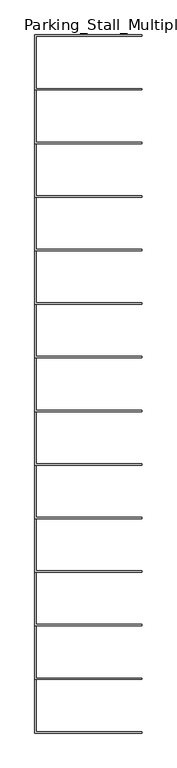
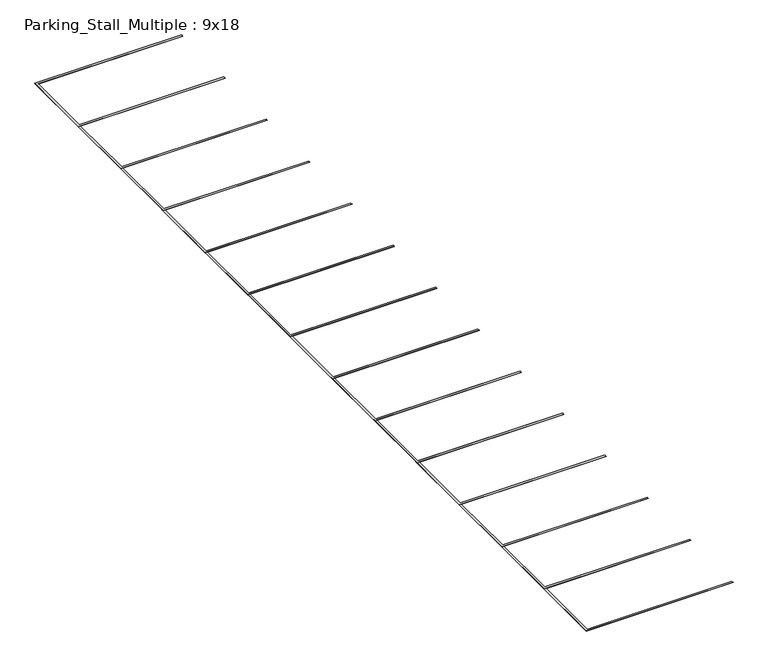
"""IFC4 building model written with IfcOpenShell, lengths in millimetres: proxy geometry, Parking_Stall_Multiple : 9x18."""

from ifc_helpers import new_model, si_unit, origin, origin_with_axes, place, context, project, spatial, polyline, outline, extrude, source, transform, mapped, element, save


def parking_stall_multiple_9x18_8b25bb00(model_context):
    return source(origin(), model_context, "Body", "SweptSolid", [
        extrude(outline(polyline([(5486.4, 32918.4), (0.0, 32918.4), (0.0, 35737.8), (5486.4, 35737.8), (5486.4, 35661.6), (76.2, 35661.6), (76.2, 32994.6), (5486.4, 32994.6), (5486.4, 32918.4)])), origin_with_axes(), (0.0, 0.0, 1.0), 6.35),
        extrude(outline(polyline([(5486.4, 30175.2), (0.0, 30175.2), (0.0, 32994.6), (5486.4, 32994.6), (5486.4, 32918.4), (76.2, 32918.4), (76.2, 30251.4), (5486.4, 30251.4), (5486.4, 30175.2)])), origin_with_axes(), (0.0, 0.0, 1.0), 6.35),
        extrude(outline(polyline([(5486.4, 27432.0), (0.0, 27432.0), (0.0, 30251.4), (5486.4, 30251.4), (5486.4, 30175.2), (76.2, 30175.2), (76.2, 27508.2), (5486.4, 27508.2), (5486.4, 27432.0)])), origin_with_axes(), (0.0, 0.0, 1.0), 6.35),
        extrude(outline(polyline([(5486.4, 24688.8), (0.0, 24688.8), (0.0, 27508.2), (5486.4, 27508.2), (5486.4, 27432.0), (76.2, 27432.0), (76.2, 24765.0), (5486.4, 24765.0), (5486.4, 24688.8)])), origin_with_axes(), (0.0, 0.0, 1.0), 6.35),
        extrude(outline(polyline([(5486.4, 21945.6), (0.0, 21945.6), (0.0, 24765.0), (5486.4, 24765.0), (5486.4, 24688.8), (76.2, 24688.8), (76.2, 22021.8), (5486.4, 22021.8), (5486.4, 21945.6)])), origin_with_axes(), (0.0, 0.0, 1.0), 6.35),
        extrude(outline(polyline([(5486.4, 19202.4), (0.0, 19202.4), (0.0, 22021.8), (5486.4, 22021.8), (5486.4, 21945.6), (76.2, 21945.6), (76.2, 19278.6), (5486.4, 19278.6), (5486.4, 19202.4)])), origin_with_axes(), (0.0, 0.0, 1.0), 6.35),
        extrude(outline(polyline([(5486.4, 16459.2), (0.0, 16459.2), (0.0, 19278.6), (5486.4, 19278.6), (5486.4, 19202.4), (76.2, 19202.4), (76.2, 16535.4), (5486.4, 16535.4), (5486.4, 16459.2)])), origin_with_axes(), (0.0, 0.0, 1.0), 6.35),
        extrude(outline(polyline([(5486.4, 13716.0), (0.0, 13716.0), (0.0, 16535.4), (5486.4, 16535.4), (5486.4, 16459.2), (76.2, 16459.2), (76.2, 13792.2), (5486.4, 13792.2), (5486.4, 13716.0)])), origin_with_axes(), (0.0, 0.0, 1.0), 6.35),
        extrude(outline(polyline([(5486.4, 10972.8), (0.0, 10972.8), (0.0, 13792.2), (5486.4, 13792.2), (5486.4, 13716.0), (76.2, 13716.0), (76.2, 11049.0), (5486.4, 11049.0), (5486.4, 10972.8)])), origin_with_axes(), (0.0, 0.0, 1.0), 6.35),
        extrude(outline(polyline([(5486.4, 8229.6), (0.0, 8229.6), (0.0, 11049.0), (5486.4, 11049.0), (5486.4, 10972.8), (76.2, 10972.8), (76.2, 8305.8), (5486.4, 8305.8), (5486.4, 8229.6)])), origin_with_axes(), (0.0, 0.0, 1.0), 6.35),
        extrude(outline(polyline([(5486.4, 5486.4), (0.0, 5486.4), (0.0, 8305.8), (5486.4, 8305.8), (5486.4, 8229.6), (76.2, 8229.6), (76.2, 5562.6), (5486.4, 5562.6), (5486.4, 5486.4)])), origin_with_axes(), (0.0, 0.0, 1.0), 6.35),
        extrude(outline(polyline([(5486.4, 2743.2), (0.0, 2743.2), (0.0, 5562.6), (5486.4, 5562.6), (5486.4, 5486.4), (76.2, 5486.4), (76.2, 2819.4), (5486.4, 2819.4), (5486.4, 2743.2)])), origin_with_axes(), (0.0, 0.0, 1.0), 6.35),
        extrude(outline(polyline([(5486.4, 0.0), (0.0, 0.0), (0.0, 2819.4), (5486.4, 2819.4), (5486.4, 2743.2), (76.2, 2743.2), (76.2, 76.2), (5486.4, 76.2), (5486.4, 0.0)])), origin_with_axes(), (0.0, 0.0, 1.0), 6.35),
    ])


if __name__ == "__main__":
    model = new_model("IFC4")
    model_context = context("Model", 3, world=origin())
    ifc_project = project(units=[si_unit("LENGTHUNIT", "METRE", prefix="MILLI")], contexts=[model_context])
    site = spatial("IfcSite", under=ifc_project)
    building = spatial("IfcBuilding", under=site)
    placement = place(None, origin())
    parking_stall_multiple_9x18_shape = parking_stall_multiple_9x18_8b25bb00(model_context)
    element("IfcBuildingElementProxy", 1, Name="Parking_Stall_Multiple : 9x18", ObjectType="Parking_Stall_Multiple : 9x18", at=placement, inside=building, context=model_context, shape_type="MappedRepresentation", body=[
        mapped(parking_stall_multiple_9x18_shape, transform((0.0, 0.0, 0.0), x_axis=(1.0, 0.0, 0.0), y_axis=(0.0, 1.0, 0.0), z_axis=(0.0, 0.0, 1.0))),
    ])
    save(model, "model.ifc")

# Revit data of these elements
# Type "Parking_Stall_Multiple : 9x18"
#   Parking_Width_M = 9' - 0"
#   Parking_Run_Length [instance default] = 65' - 0"
#   Parking_Line_Width = 0' - 3"
#   Parking_Length_M = 18' - 0"
#   Single_Parking_Visibility [instance default] = no
#   Parking_ADA_Symbol = no
#   ParkingUnitsArray [instance default] = 7
#   ParkingUnits [instance default] = 7
#   Multiple_Parking_Visibility [instance default] = yes
#   Parking_Line_Material = none
# Element 1 (IfcBuildingElementProxy, "Parking_Stall_Multiple : 9x18")
#   Parking_Run_Length = 115' - 6.83078"
#   ParkingUnitsArray = 13
#   ParkingUnits = 13
